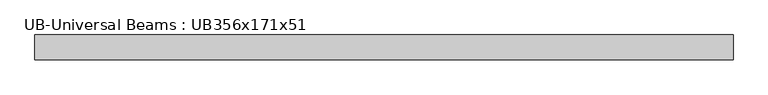
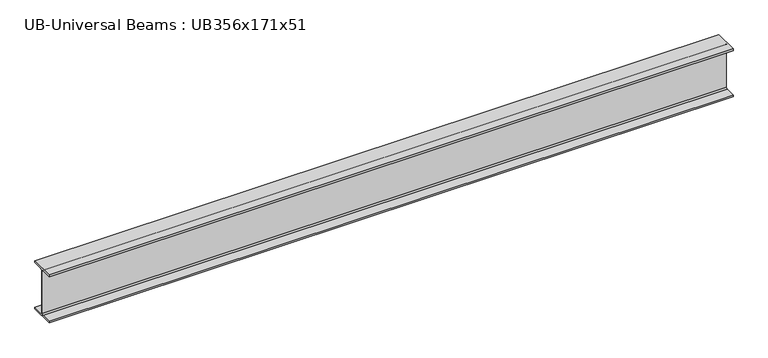
"""IFC4 building model written with IfcOpenShell, lengths in millimetres: beam geometry, UB-Universal Beams : UB356x171x51."""

from ifc_helpers import new_model, si_unit, point, frame, frame_2d, origin, place, context, project, spatial, polyline, circle_curve, trimmed, segment, composite_curve, outline, extrude, source, transform, mapped, element, save


def ub_universal_beams_ub356x171x51_eaee8fc9(model_context):
    return source(origin(), model_context, "Body", "SweptSolid", [
        extrude(outline(composite_curve([segment(polyline([(85.75, -166.0), (85.75, -177.5), (-85.75, -177.5), (-85.75, -166.0), (-13.9, -166.0)]), True, "CONTINUOUS"), segment(trimmed(circle_curve(frame_2d((-13.9, -155.8)), 10.2), [point((-13.9, -166.0))], [point((-3.7, -155.8))], True, "CARTESIAN"), True, "CONTINUOUS"), segment(polyline([(-3.7, -155.8), (-3.7, 155.8)]), True, "CONTINUOUS"), segment(trimmed(circle_curve(frame_2d((-13.9, 155.8)), 10.2), [point((-3.7, 155.8))], [point((-13.9, 166.0))], True, "CARTESIAN"), True, "CONTINUOUS"), segment(polyline([(-13.9, 166.0), (-85.75, 166.0), (-85.75, 177.5), (85.75, 177.5), (85.75, 166.0), (13.9, 166.0)]), True, "CONTINUOUS"), segment(trimmed(circle_curve(frame_2d((13.9, 155.8)), 10.2), [point((13.9, 166.0))], [point((3.7, 155.8))], True, "CARTESIAN"), True, "CONTINUOUS"), segment(polyline([(3.7, 155.8), (3.7, -155.8)]), True, "CONTINUOUS"), segment(trimmed(circle_curve(frame_2d((13.9, -155.8)), 10.2), [point((3.7, -155.8))], [point((13.9, -166.0))], True, "CARTESIAN"), True, "CONTINUOUS"), segment(polyline([(13.9, -166.0), (85.75, -166.0)]), True, "CONTINUOUS")], self_intersect=False)), frame((-2373.0, 0.0, 0.0), z_axis=(1.0, 0.0, 0.0), x_axis=(0.0, 1.0, 0.0)), (0.0, 0.0, 1.0), 4789.9),
    ])


if __name__ == "__main__":
    model = new_model("IFC4")
    model_context = context("Model", 3, world=origin())
    ifc_project = project(units=[si_unit("LENGTHUNIT", "METRE", prefix="MILLI")], contexts=[model_context])
    site = spatial("IfcSite", under=ifc_project)
    building = spatial("IfcBuilding", under=site)
    placement = place(None, origin())
    ub_universal_beams_ub356x171x51_shape = ub_universal_beams_ub356x171x51_eaee8fc9(model_context)
    element("IfcBeam", 1, ObjectType="UB-Universal Beams : UB356x171x51", at=placement, inside=building, context=model_context, shape_type="MappedRepresentation", body=[
        mapped(ub_universal_beams_ub356x171x51_shape, transform((0.0, 0.0, 0.0), x_axis=(1.0, 0.0, 0.0), y_axis=(0.0, 1.0, 0.0), z_axis=(0.0, 0.0, 1.0))),
    ])
    save(model, "model.ifc")

# Revit data of these elements
# Type "UB-Universal Beams : UB356x171x51"
#   Section Name Key = "UB356X171X51"
#   Width = 17.15 cm
#   Web Thickness = 0.74 cm
#   Web Fillet = 1.02 cm
#   Warping Constant = 286000.0 cm⁶
#   Torsional Moment of Inertia = 23.80 cm⁴
#   Section Area = 64.9 cm²
#   Plastic Modulus weak axis = 174.0 cm³
#   Plastic Modulus strong axis = 896.0 cm³
#   Nominal Weight = 50.9998 kgf/m
#   Moment of Inertia weak axis = 968.00 cm⁴
#   Moment of Inertia strong axis = 14136.00 cm⁴
#   Height = 35.5 cm
#   Flange Thickness = 1.15 cm
#   Elastic Modulus weak axis = 113.0 cm³
#   Elastic Modulus strong axis = 796.0 cm³
#   Centroid Vertical = 17.75 cm
#   Centroid Horizontal = 8.575 cm
#   Bolt Spacing = 9.0 cm
#   Length [instance default] = 1500 mm
#   Structural Material [instance default] = Metal - Steel 43-275
#   Type Comments = ""
#   Assembly Code = ""
# Element 1 (IfcBeam, "UB-Universal Beams : UB356x171x51")
#   Materials on its faces: "Metal - Steel 43-275"
# Materials
#   "Metal - Steel 43-275": class "Metal", colour RGB 247 247 247, transparency 0, Cost = 0
